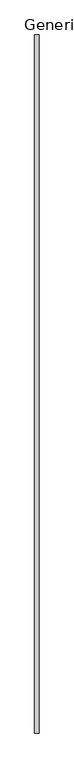
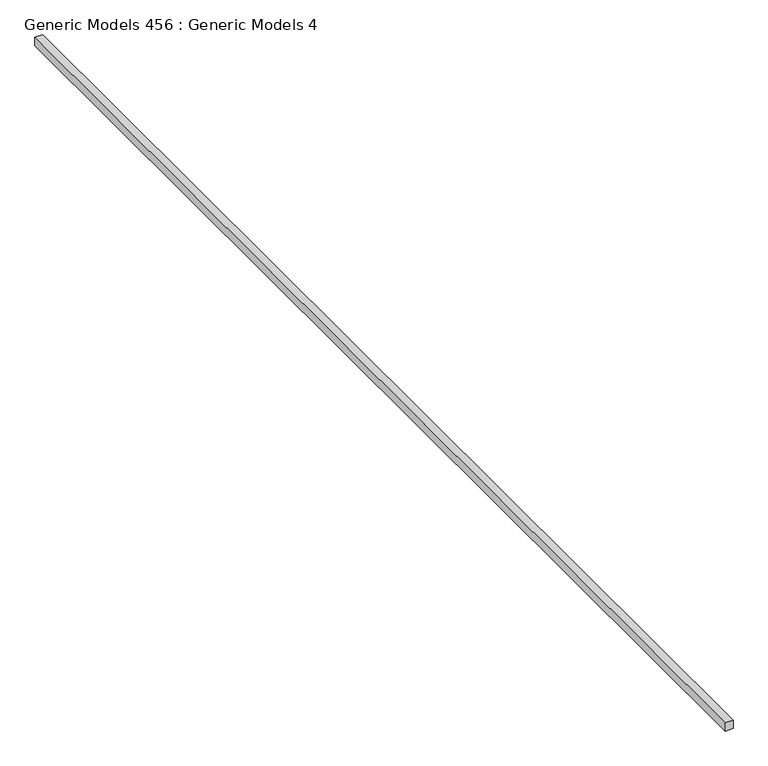
"""IFC4 building model written with IfcOpenShell, lengths in millimetres: proxy geometry, Generic Models 456 : Generic Models 4."""

from ifc_helpers import new_model, si_unit, frame, origin, place, context, project, spatial, polyline, outline, extrude, source, transform, mapped, element, save


def generic_models_456_generic_models_4_12c29e8d(model_context):
    return source(origin(), model_context, "Body", "SweptSolid", [
        extrude(outline(polyline([(1608.4513113, -6864.9230338), (1487.8013113, -6864.9230338), (1487.8013113, 11778.6769662), (1608.4513113, 11778.6769662), (1608.4513113, -6864.9230338)])), frame((0.0, 0.0, 126410.1546588), z_axis=(0.0, 0.0, 1.0), x_axis=(1.0, 0.0, 0.0)), (0.0, 0.0, 1.0), 133.6531107),
    ])


if __name__ == "__main__":
    model = new_model("IFC4")
    model_context = context("Model", 3, world=origin())
    ifc_project = project(units=[si_unit("LENGTHUNIT", "METRE", prefix="MILLI")], contexts=[model_context])
    site = spatial("IfcSite", under=ifc_project)
    building = spatial("IfcBuilding", under=site)
    placement = place(None, origin())
    generic_models_456_generic_models_4_shape = generic_models_456_generic_models_4_12c29e8d(model_context)
    element("IfcBuildingElementProxy", 1, Name="Generic Models 456 : Generic Models 4", ObjectType="Generic Models 456 : Generic Models 4", at=placement, inside=building, context=model_context, shape_type="MappedRepresentation", body=[
        mapped(generic_models_456_generic_models_4_shape, transform((0.0, 0.0, 0.0), x_axis=(1.0, 0.0, 0.0), y_axis=(0.0, 1.0, 0.0), z_axis=(0.0, 0.0, 1.0))),
    ])
    save(model, "model.ifc")

# Revit data of these elements
# Element 1 (IfcBuildingElementProxy, "Generic Models 456 : Generic Models 4")
#   Materials on its faces: "_BATT INSUL. (U-FACTOR = 0.065 MIN.) OVER CLASS II VAPOR RETARDER(TOWARD INTERIOR)"
# Materials
#   "_BATT INSUL. (U-FACTOR = 0.065 MIN.) OVER CLASS II VAPOR RETARDER(TOWARD INTERIOR)": class "Generic", colour RGB 200 166 247, transparency 0, Cost = 0
